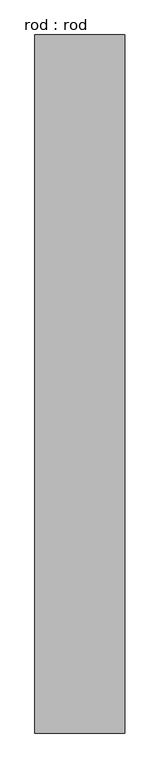
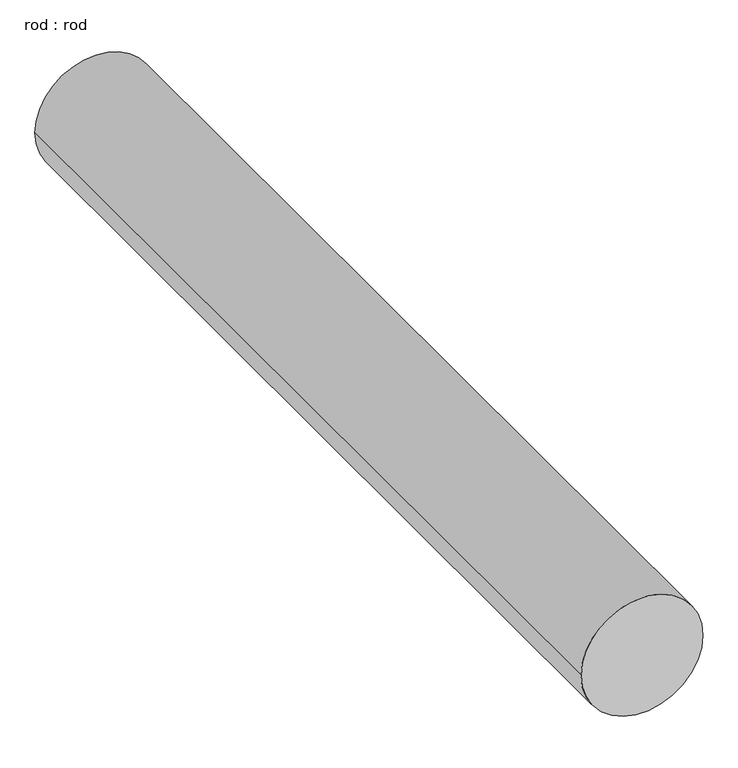
"""IFC4 building model written with IfcOpenShell, lengths in millimetres: proxy geometry, rod : rod."""

from ifc_helpers import new_model, si_unit, point, frame, frame_2d, origin, place, context, project, spatial, circle_curve, trimmed, segment, composite_curve, outline, extrude, source, transform, mapped, element, save


def rod_rod_a209afb6(model_context):
    return source(origin(), model_context, "Body", "SweptSolid", [
        extrude(outline(composite_curve([segment(trimmed(circle_curve(frame_2d((0.0108462, 0.0)), 200.0), [point((0.0108462, 200.0))], [point((0.0108462, -200.0))], False, "CARTESIAN"), True, "CONTINUOUS"), segment(trimmed(circle_curve(frame_2d((0.0108462, 0.0)), 200.0), [point((0.0108462, -200.0))], [point((0.0108462, 200.0))], False, "CARTESIAN"), True, "CONTINUOUS")], self_intersect=False)), frame((0.0, 2539.1571868, 0.0), z_axis=(0.0, 1.0, 0.0), x_axis=(0.0, 0.0, 1.0)), (0.0, 0.0, 1.0), 3107.1428571),
    ])


if __name__ == "__main__":
    model = new_model("IFC4")
    model_context = context("Model", 3, world=origin())
    ifc_project = project(units=[si_unit("LENGTHUNIT", "METRE", prefix="MILLI")], contexts=[model_context])
    site = spatial("IfcSite", under=ifc_project)
    building = spatial("IfcBuilding", under=site)
    placement = place(None, origin())
    rod_rod_shape = rod_rod_a209afb6(model_context)
    element("IfcBuildingElementProxy", 1, Name="rod : rod", ObjectType="rod : rod", at=placement, inside=building, context=model_context, shape_type="MappedRepresentation", body=[
        mapped(rod_rod_shape, transform((0.0, 0.0, 0.0), x_axis=(1.0, 0.0, 0.0), y_axis=(0.0, 1.0, 0.0), z_axis=(0.0, 0.0, 1.0))),
    ])
    save(model, "model.ifc")

# Revit data of these elements
# Type "rod : rod"
#   Default Elevation = 0
